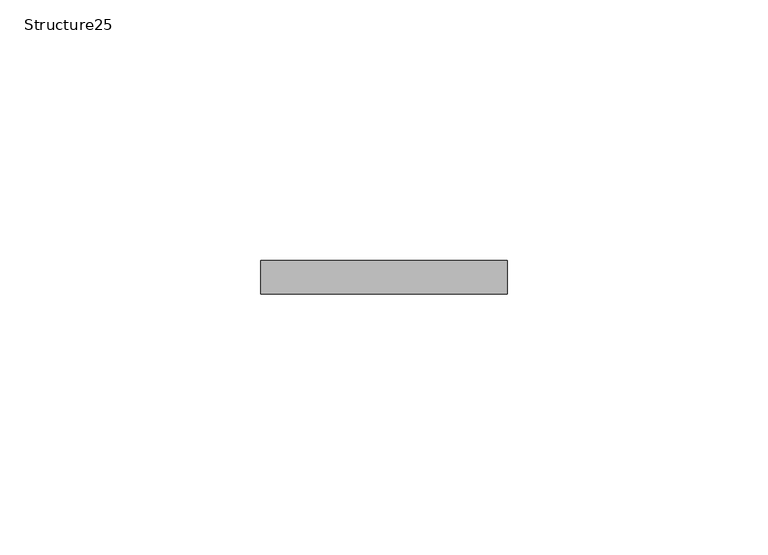
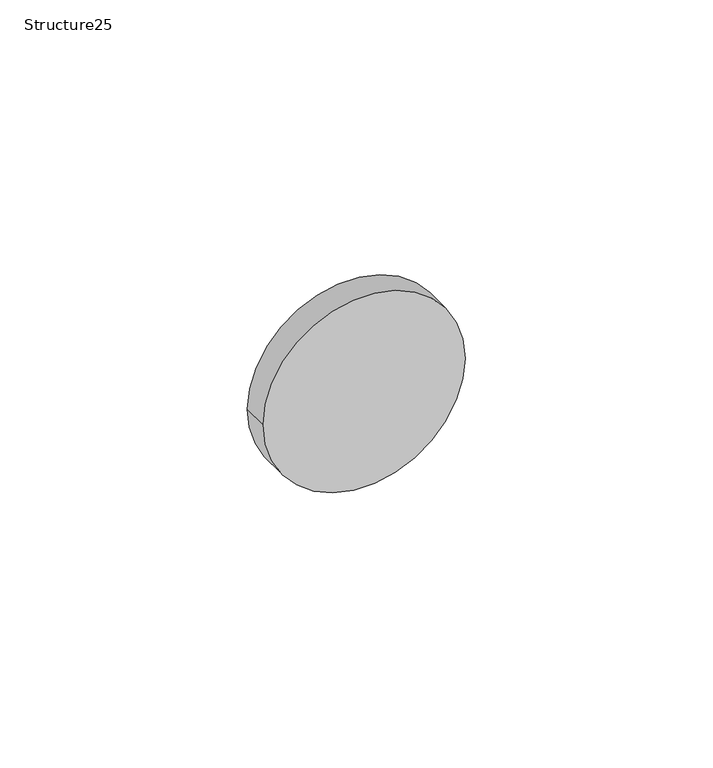
"""IFC4 building model written with IfcOpenShell, lengths in millimetres: proxy geometry, Structure25 : Structure668217153."""

from ifc_helpers import new_model, si_unit, point, frame, frame_2d, origin, place, context, project, spatial, circle_curve, trimmed, segment, composite_curve, outline, extrude, source, transform, mapped, element, save


def structure25_31314292(model_context):
    return source(origin(), model_context, "Body", "SweptSolid", [
        extrude(outline(composite_curve([segment(trimmed(circle_curve(frame_2d((40908.7088339, 9847.8795269)), 23.5716554), [point((40908.7088339, 9824.3078714))], [point((40908.7088339, 9871.4511823))], False, "CARTESIAN"), True, "CONTINUOUS"), segment(trimmed(circle_curve(frame_2d((40908.7088339, 9847.8795269)), 23.5716554), [point((40908.7088339, 9871.4511823))], [point((40908.7088339, 9824.3078714))], False, "CARTESIAN"), True, "CONTINUOUS")], self_intersect=False)), frame((0.0, 1957.9073723, 0.0), z_axis=(0.0, 1.0, 0.0), x_axis=(0.0, 0.0, 1.0)), (0.0, 0.0, 1.0), 6.35),
    ])


if __name__ == "__main__":
    model = new_model("IFC4")
    model_context = context("Model", 3, world=origin())
    ifc_project = project(units=[si_unit("LENGTHUNIT", "METRE", prefix="MILLI")], contexts=[model_context])
    site = spatial("IfcSite", under=ifc_project)
    building = spatial("IfcBuilding", under=site)
    placement = place(None, origin())
    structure25_shape = structure25_31314292(model_context)
    element("IfcBuildingElementProxy", 1, Name="Structure25 : Structure668217153", ObjectType="Structure25 : Structure668217153", at=placement, inside=building, context=model_context, shape_type="MappedRepresentation", body=[
        mapped(structure25_shape, transform((0.0, 0.0, 0.0), x_axis=(1.0, 0.0, 0.0), y_axis=(0.0, 1.0, 0.0), z_axis=(0.0, 0.0, 1.0))),
    ])
    save(model, "model.ifc")

# Revit data of these elements
# Type "Structure25 : Structure668217153"
#   NameOverride = "Structure668217153"
# Element 1 (IfcBuildingElementProxy, "Structure25 : Structure668217153")
#   Materials on its faces: "RUBBER GASKET"
# Materials
#   "RUBBER GASKET": class "Unassigned", colour RGB 70 70 70, transparency 0
